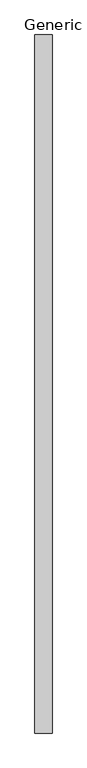
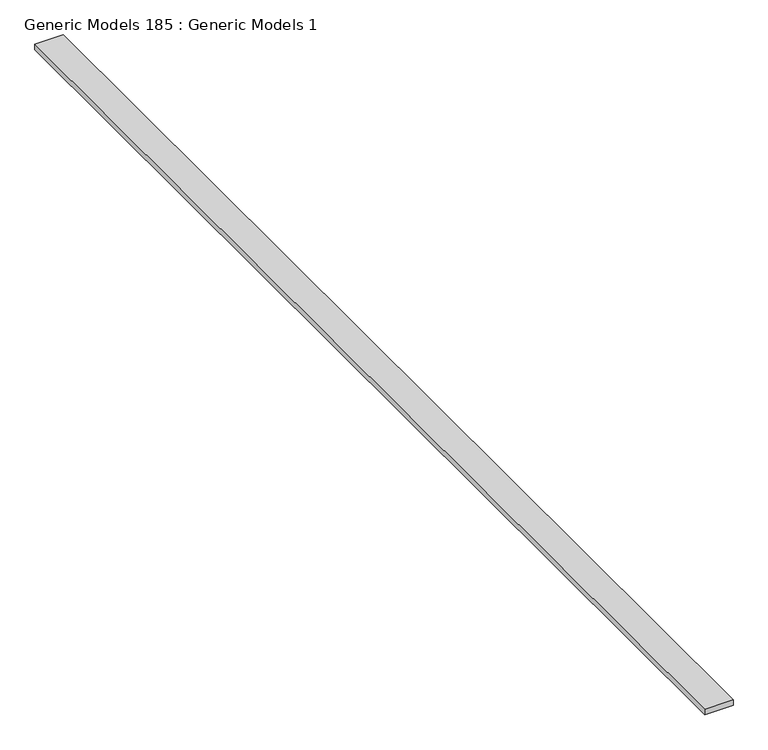
"""IFC4 building model written with IfcOpenShell, lengths in millimetres: proxy geometry, Generic Models 185 : Generic Models 1."""

from ifc_helpers import new_model, si_unit, frame, origin, place, context, project, spatial, polyline, outline, extrude, source, transform, mapped, element, save


def generic_models_185_generic_models_1_d53f1798(model_context):
    return source(origin(), model_context, "Body", "SweptSolid", [
        extrude(outline(polyline([(-5275.7536296, 7054.2769662), (-5091.6036296, 7054.2769662), (-5091.6036296, -464.1230338), (-5275.7536296, -464.1230338), (-5275.7536296, 7054.2769662)])), frame((0.0, 0.0, 126736.221), z_axis=(0.0, 0.0, 1.0), x_axis=(1.0, 0.0, 0.0)), (0.0, 0.0, 1.0), 38.1),
    ])


if __name__ == "__main__":
    model = new_model("IFC4")
    model_context = context("Model", 3, world=origin())
    ifc_project = project(units=[si_unit("LENGTHUNIT", "METRE", prefix="MILLI")], contexts=[model_context])
    site = spatial("IfcSite", under=ifc_project)
    building = spatial("IfcBuilding", under=site)
    placement = place(None, origin())
    generic_models_185_generic_models_1_shape = generic_models_185_generic_models_1_d53f1798(model_context)
    element("IfcBuildingElementProxy", 1, Name="Generic Models 185 : Generic Models 1", ObjectType="Generic Models 185 : Generic Models 1", at=placement, inside=building, context=model_context, shape_type="MappedRepresentation", body=[
        mapped(generic_models_185_generic_models_1_shape, transform((0.0, 0.0, 0.0), x_axis=(1.0, 0.0, 0.0), y_axis=(0.0, 1.0, 0.0), z_axis=(0.0, 0.0, 1.0))),
    ])
    save(model, "model.ifc")

# Revit data of these elements
# Element 1 (IfcBuildingElementProxy, "Generic Models 185 : Generic Models 1")
#   Materials on its faces: "_2X BLOCKING AS REQUIRED"
# Materials
#   "_2X BLOCKING AS REQUIRED": class "Generic", colour RGB 177 130 114, transparency 0, Cost = 0
